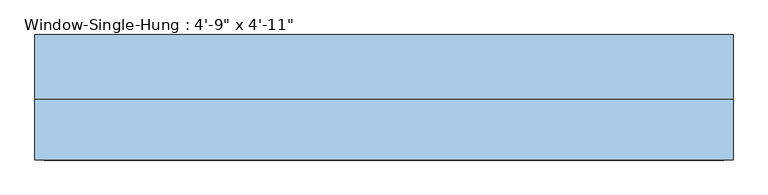
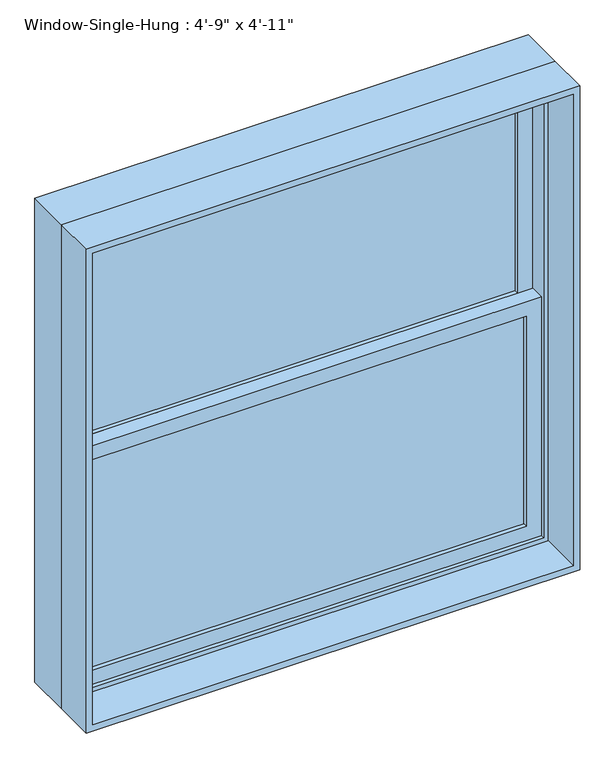
"""IFC4 building model written with IfcOpenShell, lengths in millimetres: window geometry."""

import ifcopenshell
import ifcopenshell.guid

model = None  # the IFC model being written
_history = None  # IfcOwnerHistory: only IFC2X3 demands one
_inside = {}  # id of a spatial element -> (the spatial element, [elements in it])
_under = {}  # id of a project, library or spatial element -> (it, [spatial elements below it])
_declared = {}  # id of a project -> (the project, [libraries it declares])
_typed = {}  # id of a type object -> (the type object, [elements of that type])
_made_of = {}  # id of a material, layer set ... -> (it, [elements and type objects made of it])


def new_model(schema):
    """Start an empty IFC model of exactly this schema.

    Asked for "IFC4X3", IfcOpenShell would pick the latest addendum, in which some entities
    have other attributes; the version numbers below select the first issue.
    IFC2X3 requires an IfcOwnerHistory on every rooted entity: one is made here for all.
    """
    global model, _history
    if schema == "IFC4X3":
        model = ifcopenshell.file(schema_version=(4, 3, 0, 0))
    else:
        model = ifcopenshell.file(schema=schema)
    _inside.clear()
    _under.clear()
    _declared.clear()
    _typed.clear()
    _made_of.clear()
    _history = None
    if model.schema == "IFC2X3":
        org = make("IfcOrganization", Name="unknown")
        user = make(
            "IfcPersonAndOrganization",
            ThePerson=make("IfcPerson", FamilyName="unknown"),
            TheOrganization=org,
        )
        app = make(
            "IfcApplication",
            ApplicationDeveloper=org,
            Version="unknown",
            ApplicationFullName="unknown",
            ApplicationIdentifier="unknown",
        )
        _history = make(
            "IfcOwnerHistory",
            OwningUser=user,
            OwningApplication=app,
            ChangeAction="ADDED",
            CreationDate=0,
        )
    return model


def make(cls, **values):
    """One entity of the class cls with the attributes given. An attribute that is None is left unset."""
    return model.create_entity(
        cls, **{name: value for name, value in values.items() if value is not None}
    )


def rooted(cls, **values):
    """An entity with a GlobalId (a new one), such as an element, a storey or a relation."""
    return make(cls, GlobalId=ifcopenshell.guid.new(), OwnerHistory=_history, **values)


def si_unit(unit_type, name, prefix=None):
    """IfcSIUnit, for example si_unit("LENGTHUNIT", "METRE", prefix="MILLI")."""
    return make("IfcSIUnit", UnitType=unit_type, Prefix=prefix, Name=name)


def assignment(units):
    """IfcUnitAssignment: the units of a project."""
    return None if units is None else make("IfcUnitAssignment", Units=units)


def point(xyz):
    """IfcCartesianPoint."""
    return None if xyz is None else make("IfcCartesianPoint", Coordinates=xyz)


def direction(xyz):
    """IfcDirection."""
    return None if xyz is None else make("IfcDirection", DirectionRatios=xyz)


def frame(location, z_axis=None, x_axis=None):
    """IfcAxis2Placement3D, a coordinate frame: its origin and axes. An axis left out is left unset."""
    return make(
        "IfcAxis2Placement3D",
        Location=point(location),
        Axis=direction(z_axis),
        RefDirection=direction(x_axis),
    )


def origin():
    """The frame at (0, 0, 0) with its axes left unset."""
    return frame((0.0, 0.0, 0.0))


def place(relative_to, where):
    """IfcLocalPlacement: puts the frame where relative to a parent placement (None: the world)."""
    return make(
        "IfcLocalPlacement", PlacementRelTo=relative_to, RelativePlacement=where
    )


def context(
    kind, dimensions, precision=None, world=None, true_north=None, identifier=None
):
    """IfcGeometricRepresentationContext, for example the 3D "Model" context."""
    return make(
        "IfcGeometricRepresentationContext",
        ContextIdentifier=identifier,
        ContextType=kind,
        CoordinateSpaceDimension=dimensions,
        Precision=precision,
        WorldCoordinateSystem=world,
        TrueNorth=true_north,
    )


def project(units=None, contexts=None):
    """IfcProject with its units and contexts."""
    return rooted(
        "IfcProject",
        Name="project",
        RepresentationContexts=contexts,
        UnitsInContext=assignment(units),
    )


def spatial(cls, under=None, at=None, **own):
    """A site, building, storey or space (cls), placed at a placement, below another one or the project."""
    s = rooted(cls, ObjectPlacement=at, **own)
    if under is not None:
        _under.setdefault(under.id(), (under, []))[1].append(s)
    return s


def polyline(points):
    """IfcPolyline through the points."""
    return make("IfcPolyline", Points=[point(p) for p in points])


def outline(outer, holes=None, kind="AREA"):
    """IfcArbitraryClosedProfileDef: a profile drawn as a closed curve; with holes, ...WithVoids."""
    if holes is None:
        return make("IfcArbitraryClosedProfileDef", ProfileType=kind, OuterCurve=outer)
    return make(
        "IfcArbitraryProfileDefWithVoids",
        ProfileType=kind,
        OuterCurve=outer,
        InnerCurves=holes,
    )


def extrude(swept, where, along, depth):
    """IfcExtrudedAreaSolid: the profile swept, set in the frame where, extruded along a direction by depth."""
    return make(
        "IfcExtrudedAreaSolid",
        SweptArea=swept,
        Position=where,
        ExtrudedDirection=direction(along),
        Depth=depth,
    )


def shape(context_of_items, identifier, shape_type, items):
    """IfcShapeRepresentation: the items that make up one representation, for example the "Body"."""
    return make(
        "IfcShapeRepresentation",
        ContextOfItems=context_of_items,
        RepresentationIdentifier=identifier,
        RepresentationType=shape_type,
        Items=items,
    )


def source(mapping_origin, context_of_items, identifier, shape_type, items):
    """IfcRepresentationMap: a shape defined once, which mapped items show again and again."""
    return make(
        "IfcRepresentationMap",
        MappingOrigin=mapping_origin,
        MappedRepresentation=shape(context_of_items, identifier, shape_type, items),
    )


def transform(
    local_origin,
    x_axis=None,
    y_axis=None,
    z_axis=None,
    scale=None,
    scale2=None,
    scale3=None,
    uniform=True,
):
    """IfcCartesianTransformationOperator3D, or its non-uniform kind. x_axis, y_axis, z_axis: its Axis1, 2, 3."""
    if uniform:
        return make(
            "IfcCartesianTransformationOperator3D",
            Axis1=direction(x_axis),
            Axis2=direction(y_axis),
            LocalOrigin=point(local_origin),
            Scale=scale,
            Axis3=direction(z_axis),
        )
    return make(
        "IfcCartesianTransformationOperator3DnonUniform",
        Axis1=direction(x_axis),
        Axis2=direction(y_axis),
        LocalOrigin=point(local_origin),
        Scale=scale,
        Axis3=direction(z_axis),
        Scale2=scale2,
        Scale3=scale3,
    )


def mapped(mapping_source, mapping_target):
    """IfcMappedItem: shows the shape of a source again, moved by a transform."""
    return make(
        "IfcMappedItem", MappingSource=mapping_source, MappingTarget=mapping_target
    )


def made_of(thing, what):
    """Note that an element or type object is made of a material, layer set ...; save() writes the relation."""
    if what is not None:
        _made_of.setdefault(what.id(), (what, []))[1].append(thing)
    return thing


def element(
    cls,
    number,
    at=None,
    inside=None,
    cuts=None,
    type_object=None,
    material=None,
    context=None,
    identifier="Body",
    shape_type=None,
    held_by="IfcProductDefinitionShape",
    body=None,
    shapes=None,
    **own,
):
    """One element of the class cls, such as IfcWall. Its Tag is "e" and its number.

    at: its placement. inside: the storey or other place that contains it. cuts: it is an
    opening in that element (IfcRelVoidsElement). A single representation is given by context,
    identifier, shape_type and body (its items); several are given by shapes. held_by: the class
    of the entity that holds the representations. save() writes the other relations.
    """
    e = rooted(cls, Tag="e%d" % number, ObjectPlacement=at, **own)
    if body is not None:
        shapes = [shape(context, identifier, shape_type, body)]
    if shapes is not None:
        e.Representation = make(held_by, Representations=shapes)
    if inside is not None:
        _inside.setdefault(inside.id(), (inside, []))[1].append(e)
    if cuts is not None:
        rooted(
            "IfcRelVoidsElement", RelatingBuildingElement=cuts, RelatedOpeningElement=e
        )
    if type_object is not None:
        _typed.setdefault(type_object.id(), (type_object, []))[1].append(e)
    return made_of(e, material)


def aggregate(whole, parts):
    """IfcRelAggregates: a whole, such as a stair, and the parts it consists of."""
    return rooted("IfcRelAggregates", RelatingObject=whole, RelatedObjects=parts)


def save(model, path):
    """Write the relations noted so far, then the file.

    IfcRelAggregates (storeys below a building ...), IfcRelContainedInSpatialStructure (elements
    in a storey), IfcRelDefinesByType, IfcRelAssociatesMaterial and IfcRelDeclares: one each for
    every whole, place, type object, material and project.
    """
    for whole, parts in _under.values():
        aggregate(whole, parts)
    for where, things in _inside.values():
        rooted(
            "IfcRelContainedInSpatialStructure",
            RelatedElements=things,
            RelatingStructure=where,
        )
    for kind, things in _typed.values():
        rooted("IfcRelDefinesByType", RelatedObjects=things, RelatingType=kind)
    for what, things in _made_of.values():
        rooted("IfcRelAssociatesMaterial", RelatedObjects=things, RelatingMaterial=what)
    for by, libraries in _declared.values():
        rooted("IfcRelDeclares", RelatingContext=by, RelatedDefinitions=libraries)
    model.write(path)


def window_55bfdad2(model_context):
    return source(origin(), model_context, "Body", "SweptSolid", [
        extrude(outline(polyline([(647.7, 50.8), (647.7, 44.45), (-647.7, 44.45), (-647.7, 50.8), (647.7, 50.8)])), frame((0.0, 0.0, 990.6), z_axis=(0.0, 0.0, 1.0), x_axis=(1.0, 0.0, 0.0)), (0.0, 0.0, 1.0), 650.875),
        extrude(outline(polyline([(-647.7, 38.1), (647.7, 38.1), (647.7, 31.75), (-647.7, 31.75), (-647.7, 38.1)])), frame((0.0, 0.0, 990.6), z_axis=(0.0, 0.0, 1.0), x_axis=(1.0, 0.0, 0.0)), (0.0, 0.0, 1.0), 650.875),
        extrude(outline(polyline([(647.7, 95.25), (647.7, 88.9), (-647.7, 88.9), (-647.7, 95.25), (647.7, 95.25)])), frame((0.0, 0.0, 1685.925), z_axis=(0.0, 0.0, 1.0), x_axis=(1.0, 0.0, 0.0)), (0.0, 0.0, 1.0), 650.875),
        extrude(outline(polyline([(-647.7, 82.55), (647.7, 82.55), (647.7, 76.2), (-647.7, 76.2), (-647.7, 82.55)])), frame((0.0, 0.0, 1685.925), z_axis=(0.0, 0.0, 1.0), x_axis=(1.0, 0.0, 0.0)), (0.0, 0.0, 1.0), 650.875),
        extrude(outline(polyline([(1685.925, -692.15), (946.15, -692.15), (946.15, 692.15), (1685.925, 692.15), (1685.925, -692.15)]), holes=[polyline([(1641.475, 647.7), (990.6, 647.7), (990.6, -647.7), (1641.475, -647.7), (1641.475, 647.7)])]), frame((0.0, 19.05, 0.0), z_axis=(0.0, 1.0, 0.0), x_axis=(0.0, 0.0, 1.0)), (0.0, 0.0, 1.0), 44.45),
        extrude(outline(polyline([(2381.25, -692.15), (1641.475, -692.15), (1641.475, 692.15), (2381.25, 692.15), (2381.25, -692.15)]), holes=[polyline([(2336.8, 647.7), (1685.925, 647.7), (1685.925, -647.7), (2336.8, -647.7), (2336.8, 647.7)])]), frame((0.0, 63.5, 0.0), z_axis=(0.0, 1.0, 0.0), x_axis=(0.0, 0.0, 1.0)), (0.0, 0.0, 1.0), 44.45),
        extrude(outline(polyline([(2413.0, -723.9), (914.4, -723.9), (914.4, 723.9), (2413.0, 723.9), (2413.0, -723.9)]), holes=[polyline([(2381.25, 692.15), (946.15, 692.15), (946.15, -692.15), (2381.25, -692.15), (2381.25, 692.15)])]), frame((0.0, 6.35, 0.0), z_axis=(0.0, 1.0, 0.0), x_axis=(0.0, 0.0, 1.0)), (0.0, 0.0, 1.0), 133.35),
        extrude(outline(polyline([(2413.0, 723.9), (2413.0, -723.9), (914.4, -723.9), (914.4, 723.9), (2413.0, 723.9)]), holes=[polyline([(2393.95, 704.85), (933.45, 704.85), (933.45, -704.85), (2393.95, -704.85), (2393.95, 704.85)])]), frame((0.0, -120.65, 0.0), z_axis=(0.0, 1.0, 0.0), x_axis=(0.0, 0.0, 1.0)), (0.0, 0.0, 1.0), 127.0),
    ])


if __name__ == "__main__":
    model = new_model("IFC4")
    model_context = context("Model", 3, world=origin())
    ifc_project = project(units=[si_unit("LENGTHUNIT", "METRE", prefix="MILLI")], contexts=[model_context])
    site = spatial("IfcSite", under=ifc_project)
    building = spatial("IfcBuilding", under=site)
    placement = place(None, origin())
    window_shape = window_55bfdad2(model_context)
    element("IfcWindow", 1, ObjectType="Window-Single-Hung : 4'-9\" x 4'-11\"", at=placement, inside=building, context=model_context, shape_type="MappedRepresentation", body=[
        mapped(window_shape, transform((0.0, 0.0, 0.0), x_axis=(1.0, 0.0, 0.0), y_axis=(0.0, 1.0, 0.0), z_axis=(0.0, 0.0, 1.0))),
    ])
    save(model, "model.ifc")

# Revit data of these elements
# Type "Window-Single-Hung : 4'-9\" x 4'-11\""
#   Type Mark = "23"
#   Fire Rating = "0.5h"
#   Construction Type Id = "DG-DR"
#   Assembly Code = "B2020100"
#   Analytic Construction = "Double glazing - domestic"
#   Wall Thickness [instance default] = 0' - 6"
#   Window Inset [instance default] = 0' - 0"
#   Visual Light Transmittance = 0.81
#   Thermal Resistance (R) = 0.319569 (m²·K)/W
#   Solar Heat Gain Coefficient = 0.76
#   Muntin Width = 4' - 3"
#   Muntin Height = 2' - 1 5/8"
#   Interior Wall Closure [instance default] = 0' - 1 1/2"
#   Rough Width = 4' - 9 1/2"
#   Rough Height = 4' - 11 1/2"
#   Frame Extension [instance default] = 0' - 1 1/4"
#   Exterior Wall Closure [instance default] = 0' - 0 1/2"
#   Extension Jamb [instance default] = 0' - 1 1/2"
#   Heat Transfer Coefficient (U) = 3.12929 W/(m²·K)
#   Height = 4' - 11"
#   Width = 4' - 9"
#   Top Muntin Visibility = no
#   Indicator Visibility = no
#   Extension Jamb Visibility [instance default] = yes
#   Interior Trim Visibility [instance default] = yes
#   Exterior Trim Visibility [instance default] = yes
#   Bottom Muntin Visibility = no
#   Muntin Pattern = Muntin Pattern_2x2 : Muntin Pattern_2x2
#   Interior Trim Material = Wood - Stained
#   Interior Trim = Trim-Window-Interior-Flat : Picture Frame
#   Exterior Trim Material = Clad - White
#   Exterior Trim = Trim-Window-Exterior-Flat : with Sill
#   Glass Panel Material = Glass
#   Exterior Frame Material = Clad - White
#   Interior Frame Material = Wood - Stained
#   Wall Closure = (empty or 0)
# Element 1 (IfcWindow, "Window-Single-Hung : 4'-9\" x 4'-11\"")
#   Wall Thickness = 0' - 9 1/2"
#   Extension Jamb = 0' - 5"
#   Materials on its faces: "Wood - Stained", "Glass", "Clad - White"
# Materials
#   "Wood - Stained": class "Wood", colour RGB 224 178 126, transparency 0, Cost = 0
#   "Clad - White": class "Wood", colour RGB 242 242 238, transparency 0, Cost = 0
#   "Glass": class "Glass", colour RGB 218 227 224, transparency 0.85, Description = "Soda Lime Glass", Cost = 0
